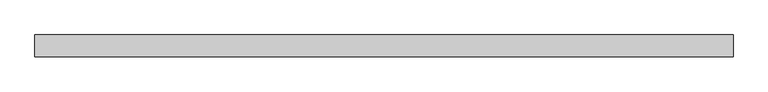
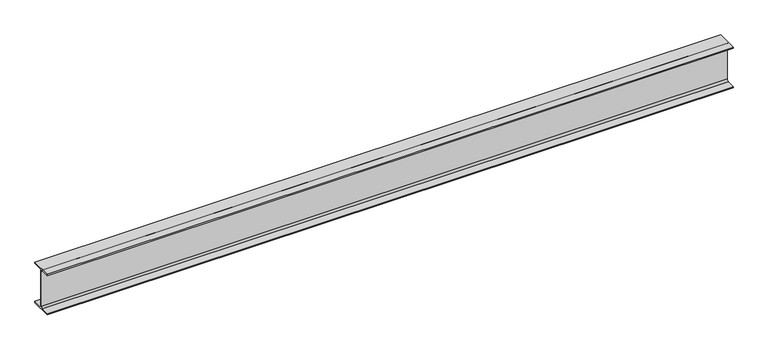
"""IFC4 building model written with IfcOpenShell, lengths in millimetres: beam geometry, 0912_Steel Framing_H-KSD3502 : H_SB_AR_S02_H-300x150x6.5x9_Stair."""

import ifcopenshell
import ifcopenshell.guid

model = None  # the IFC model being written
_history = None  # IfcOwnerHistory: only IFC2X3 demands one
_inside = {}  # id of a spatial element -> (the spatial element, [elements in it])
_under = {}  # id of a project, library or spatial element -> (it, [spatial elements below it])
_declared = {}  # id of a project -> (the project, [libraries it declares])
_typed = {}  # id of a type object -> (the type object, [elements of that type])
_made_of = {}  # id of a material, layer set ... -> (it, [elements and type objects made of it])


def new_model(schema):
    """Start an empty IFC model of exactly this schema.

    Asked for "IFC4X3", IfcOpenShell would pick the latest addendum, in which some entities
    have other attributes; the version numbers below select the first issue.
    IFC2X3 requires an IfcOwnerHistory on every rooted entity: one is made here for all.
    """
    global model, _history
    if schema == "IFC4X3":
        model = ifcopenshell.file(schema_version=(4, 3, 0, 0))
    else:
        model = ifcopenshell.file(schema=schema)
    _inside.clear()
    _under.clear()
    _declared.clear()
    _typed.clear()
    _made_of.clear()
    _history = None
    if model.schema == "IFC2X3":
        org = make("IfcOrganization", Name="unknown")
        user = make(
            "IfcPersonAndOrganization",
            ThePerson=make("IfcPerson", FamilyName="unknown"),
            TheOrganization=org,
        )
        app = make(
            "IfcApplication",
            ApplicationDeveloper=org,
            Version="unknown",
            ApplicationFullName="unknown",
            ApplicationIdentifier="unknown",
        )
        _history = make(
            "IfcOwnerHistory",
            OwningUser=user,
            OwningApplication=app,
            ChangeAction="ADDED",
            CreationDate=0,
        )
    return model


def make(cls, **values):
    """One entity of the class cls with the attributes given. An attribute that is None is left unset."""
    return model.create_entity(
        cls, **{name: value for name, value in values.items() if value is not None}
    )


def rooted(cls, **values):
    """An entity with a GlobalId (a new one), such as an element, a storey or a relation."""
    return make(cls, GlobalId=ifcopenshell.guid.new(), OwnerHistory=_history, **values)


def si_unit(unit_type, name, prefix=None):
    """IfcSIUnit, for example si_unit("LENGTHUNIT", "METRE", prefix="MILLI")."""
    return make("IfcSIUnit", UnitType=unit_type, Prefix=prefix, Name=name)


def assignment(units):
    """IfcUnitAssignment: the units of a project."""
    return None if units is None else make("IfcUnitAssignment", Units=units)


def point(xyz):
    """IfcCartesianPoint."""
    return None if xyz is None else make("IfcCartesianPoint", Coordinates=xyz)


def direction(xyz):
    """IfcDirection."""
    return None if xyz is None else make("IfcDirection", DirectionRatios=xyz)


def frame(location, z_axis=None, x_axis=None):
    """IfcAxis2Placement3D, a coordinate frame: its origin and axes. An axis left out is left unset."""
    return make(
        "IfcAxis2Placement3D",
        Location=point(location),
        Axis=direction(z_axis),
        RefDirection=direction(x_axis),
    )


def frame_2d(location, x_axis=None):
    """IfcAxis2Placement2D, a coordinate frame in the plane: its origin and x axis."""
    return make(
        "IfcAxis2Placement2D", Location=point(location), RefDirection=direction(x_axis)
    )


def origin():
    """The frame at (0, 0, 0) with its axes left unset."""
    return frame((0.0, 0.0, 0.0))


def place(relative_to, where):
    """IfcLocalPlacement: puts the frame where relative to a parent placement (None: the world)."""
    return make(
        "IfcLocalPlacement", PlacementRelTo=relative_to, RelativePlacement=where
    )


def context(
    kind, dimensions, precision=None, world=None, true_north=None, identifier=None
):
    """IfcGeometricRepresentationContext, for example the 3D "Model" context."""
    return make(
        "IfcGeometricRepresentationContext",
        ContextIdentifier=identifier,
        ContextType=kind,
        CoordinateSpaceDimension=dimensions,
        Precision=precision,
        WorldCoordinateSystem=world,
        TrueNorth=true_north,
    )


def project(units=None, contexts=None):
    """IfcProject with its units and contexts."""
    return rooted(
        "IfcProject",
        Name="project",
        RepresentationContexts=contexts,
        UnitsInContext=assignment(units),
    )


def spatial(cls, under=None, at=None, **own):
    """A site, building, storey or space (cls), placed at a placement, below another one or the project."""
    s = rooted(cls, ObjectPlacement=at, **own)
    if under is not None:
        _under.setdefault(under.id(), (under, []))[1].append(s)
    return s


def polyline(points):
    """IfcPolyline through the points."""
    return make("IfcPolyline", Points=[point(p) for p in points])


def circle_curve(where, radius):
    """IfcCircle in the frame where."""
    return make("IfcCircle", Position=where, Radius=radius)


def trimmed(basis, trim1, trim2, sense, master):
    """IfcTrimmedCurve: the piece of a basis curve between two trims."""
    return make(
        "IfcTrimmedCurve",
        BasisCurve=basis,
        Trim1=trim1,
        Trim2=trim2,
        SenseAgreement=sense,
        MasterRepresentation=master,
    )


def segment(curve, same_sense, transition):
    """IfcCompositeCurveSegment."""
    return make(
        "IfcCompositeCurveSegment",
        Transition=transition,
        SameSense=same_sense,
        ParentCurve=curve,
    )


def composite_curve(segments, self_intersect=None):
    """IfcCompositeCurve: segments joined end to end."""
    return make("IfcCompositeCurve", Segments=segments, SelfIntersect=self_intersect)


def outline(outer, holes=None, kind="AREA"):
    """IfcArbitraryClosedProfileDef: a profile drawn as a closed curve; with holes, ...WithVoids."""
    if holes is None:
        return make("IfcArbitraryClosedProfileDef", ProfileType=kind, OuterCurve=outer)
    return make(
        "IfcArbitraryProfileDefWithVoids",
        ProfileType=kind,
        OuterCurve=outer,
        InnerCurves=holes,
    )


def extrude(swept, where, along, depth):
    """IfcExtrudedAreaSolid: the profile swept, set in the frame where, extruded along a direction by depth."""
    return make(
        "IfcExtrudedAreaSolid",
        SweptArea=swept,
        Position=where,
        ExtrudedDirection=direction(along),
        Depth=depth,
    )


def shape(context_of_items, identifier, shape_type, items):
    """IfcShapeRepresentation: the items that make up one representation, for example the "Body"."""
    return make(
        "IfcShapeRepresentation",
        ContextOfItems=context_of_items,
        RepresentationIdentifier=identifier,
        RepresentationType=shape_type,
        Items=items,
    )


def source(mapping_origin, context_of_items, identifier, shape_type, items):
    """IfcRepresentationMap: a shape defined once, which mapped items show again and again."""
    return make(
        "IfcRepresentationMap",
        MappingOrigin=mapping_origin,
        MappedRepresentation=shape(context_of_items, identifier, shape_type, items),
    )


def transform(
    local_origin,
    x_axis=None,
    y_axis=None,
    z_axis=None,
    scale=None,
    scale2=None,
    scale3=None,
    uniform=True,
):
    """IfcCartesianTransformationOperator3D, or its non-uniform kind. x_axis, y_axis, z_axis: its Axis1, 2, 3."""
    if uniform:
        return make(
            "IfcCartesianTransformationOperator3D",
            Axis1=direction(x_axis),
            Axis2=direction(y_axis),
            LocalOrigin=point(local_origin),
            Scale=scale,
            Axis3=direction(z_axis),
        )
    return make(
        "IfcCartesianTransformationOperator3DnonUniform",
        Axis1=direction(x_axis),
        Axis2=direction(y_axis),
        LocalOrigin=point(local_origin),
        Scale=scale,
        Axis3=direction(z_axis),
        Scale2=scale2,
        Scale3=scale3,
    )


def mapped(mapping_source, mapping_target):
    """IfcMappedItem: shows the shape of a source again, moved by a transform."""
    return make(
        "IfcMappedItem", MappingSource=mapping_source, MappingTarget=mapping_target
    )


def made_of(thing, what):
    """Note that an element or type object is made of a material, layer set ...; save() writes the relation."""
    if what is not None:
        _made_of.setdefault(what.id(), (what, []))[1].append(thing)
    return thing


def element(
    cls,
    number,
    at=None,
    inside=None,
    cuts=None,
    type_object=None,
    material=None,
    context=None,
    identifier="Body",
    shape_type=None,
    held_by="IfcProductDefinitionShape",
    body=None,
    shapes=None,
    **own,
):
    """One element of the class cls, such as IfcWall. Its Tag is "e" and its number.

    at: its placement. inside: the storey or other place that contains it. cuts: it is an
    opening in that element (IfcRelVoidsElement). A single representation is given by context,
    identifier, shape_type and body (its items); several are given by shapes. held_by: the class
    of the entity that holds the representations. save() writes the other relations.
    """
    e = rooted(cls, Tag="e%d" % number, ObjectPlacement=at, **own)
    if body is not None:
        shapes = [shape(context, identifier, shape_type, body)]
    if shapes is not None:
        e.Representation = make(held_by, Representations=shapes)
    if inside is not None:
        _inside.setdefault(inside.id(), (inside, []))[1].append(e)
    if cuts is not None:
        rooted(
            "IfcRelVoidsElement", RelatingBuildingElement=cuts, RelatedOpeningElement=e
        )
    if type_object is not None:
        _typed.setdefault(type_object.id(), (type_object, []))[1].append(e)
    return made_of(e, material)


def aggregate(whole, parts):
    """IfcRelAggregates: a whole, such as a stair, and the parts it consists of."""
    return rooted("IfcRelAggregates", RelatingObject=whole, RelatedObjects=parts)


def save(model, path):
    """Write the relations noted so far, then the file.

    IfcRelAggregates (storeys below a building ...), IfcRelContainedInSpatialStructure (elements
    in a storey), IfcRelDefinesByType, IfcRelAssociatesMaterial and IfcRelDeclares: one each for
    every whole, place, type object, material and project.
    """
    for whole, parts in _under.values():
        aggregate(whole, parts)
    for where, things in _inside.values():
        rooted(
            "IfcRelContainedInSpatialStructure",
            RelatedElements=things,
            RelatingStructure=where,
        )
    for kind, things in _typed.values():
        rooted("IfcRelDefinesByType", RelatedObjects=things, RelatingType=kind)
    for what, things in _made_of.values():
        rooted("IfcRelAssociatesMaterial", RelatedObjects=things, RelatingMaterial=what)
    for by, libraries in _declared.values():
        rooted("IfcRelDeclares", RelatingContext=by, RelatedDefinitions=libraries)
    model.write(path)


def beam_fed367b4(model_context):
    return source(origin(), model_context, "Body", "SweptSolid", [
        extrude(outline(composite_curve([segment(polyline([(75.0, -141.0), (75.0, -150.0), (-75.0, -150.0), (-75.0, -141.0), (-16.25, -141.0)]), True, "CONTINUOUS"), segment(trimmed(circle_curve(frame_2d((-16.25, -128.0)), 13.0), [point((-16.25, -141.0))], [point((-3.25, -128.0))], True, "CARTESIAN"), True, "CONTINUOUS"), segment(polyline([(-3.25, -128.0), (-3.25, 128.0)]), True, "CONTINUOUS"), segment(trimmed(circle_curve(frame_2d((-16.25, 128.0)), 13.0), [point((-3.25, 128.0))], [point((-16.25, 141.0))], True, "CARTESIAN"), True, "CONTINUOUS"), segment(polyline([(-16.25, 141.0), (-75.0, 141.0), (-75.0, 150.0), (75.0, 150.0), (75.0, 141.0), (16.25, 141.0)]), True, "CONTINUOUS"), segment(trimmed(circle_curve(frame_2d((16.25, 128.0)), 13.0), [point((16.25, 141.0))], [point((3.25, 128.0))], True, "CARTESIAN"), True, "CONTINUOUS"), segment(polyline([(3.25, 128.0), (3.25, -128.0)]), True, "CONTINUOUS"), segment(trimmed(circle_curve(frame_2d((16.25, -128.0)), 13.0), [point((3.25, -128.0))], [point((16.25, -141.0))], True, "CARTESIAN"), True, "CONTINUOUS"), segment(polyline([(16.25, -141.0), (75.0, -141.0)]), True, "CONTINUOUS")], self_intersect=False)), frame((-2381.1079142, 0.0, 0.0), z_axis=(1.0, 0.0, 0.0), x_axis=(0.0, 1.0, 0.0)), (0.0, 0.0, 1.0), 4799.4668533),
    ])


if __name__ == "__main__":
    model = new_model("IFC4")
    model_context = context("Model", 3, world=origin())
    ifc_project = project(units=[si_unit("LENGTHUNIT", "METRE", prefix="MILLI")], contexts=[model_context])
    site = spatial("IfcSite", under=ifc_project)
    building = spatial("IfcBuilding", under=site)
    placement = place(None, origin())
    beam_shape = beam_fed367b4(model_context)
    element("IfcBeam", 1, ObjectType="0912_Steel Framing_H-KSD3502 : H_SB_AR_S02_H-300x150x6.5x9_Stair", at=placement, inside=building, context=model_context, shape_type="MappedRepresentation", body=[
        mapped(beam_shape, transform((0.0, 0.0, 0.0), x_axis=(1.0, 0.0, 0.0), y_axis=(0.0, 1.0, 0.0), z_axis=(0.0, 0.0, 1.0))),
    ])
    save(model, "model.ifc")

# Revit data of these elements
# Type "0912_Steel Framing_H-KSD3502 : H_SB_AR_S02_H-300x150x6.5x9_Stair"
#   H_Q'ty Cal Type Tag = "SB-Q2"
#   H_WM Code_1 = "S01AA073-00001 |  | TON | Main Steel Structure Fabrication Work | Shelter/Building | Medium Steel - Standard |  |  |  |  |  |  | Material: (   ) | (90)KG/M>Weight≥(30)KG/M | S01AA073-00001 Main Steel Structure Fabrication Work Shelter/Building Medium Steel - Standard         | - Material: ( ASTM A36 )\n- (90)KG/M>Weight≥(30)KG/M"
#   H_WM Code_2 = "S03AA083-00001 |  | TON | Main Steel Structure Erection Work | Shelter/Building | Medium Steel |  |  |  |  |  |  | Material: (   ) | S03AA083-00001 Main Steel Structure Erection Work Shelter/Building Medium Steel         | - Material: ( ASTM A36 )"
#   H_WM Code_3 = "S01AA009-00001 |  | TON | Main Steel Structure Fabrication Work | Shelter/Building | Plates - Gusset, Stiffener, ETC | Material: (   ) | S01AA009-00001 Main Steel Structure Fabrication Work Shelter/Building Plates - Gusset, Stiffener, ETC         |"
#   H_WM Code_4 = "S41AA051-00001 |  | M2 | Steel Structure Paint Work | Shelter/Building | for Non-Fireproofed Steel Surface |  |  |  |  |  |  | Material: (   ) | S41AA051-00001 Steel Structure Paint Work Shelter/Building for Non-Fireproofed Steel Surface         |"
#   Width = 15.0 cm
#   Web Thickness = 0.65 cm
#   Web Fillet = 1.3 cm
#   Warping Constant = 107000.0 cm⁶
#   W = 0
#   Torsional Moment of Inertia = 9.9539 cm⁴
#   Section Area = 46.78 cm²
#   Plastic Modulus weak axis = 105.0 cm³
#   Plastic Modulus strong axis = 542.0 cm³
#   Perimeter = 1.17 m²/m
#   Nominal Weight = 36.70 kgf/m
#   Moment of Inertia weak axis = 508.00 cm⁴
#   Moment of Inertia strong axis = 7210.00 cm⁴
#   Height = 30.0 cm
#   Flange Thickness = 0.9 cm
#   Elastic Modulus weak axis = 67.7 cm³
#   Elastic Modulus strong axis = 481.0 cm³
#   Centroid Vertical = 15.0 cm
#   Centroid Horizontal = 7.5 cm
#   Ix = 72100000
#   Length [instance default] = 1524 mm
#   Zx = 542000
#   b = 150 mm
#   h = 300 mm
#   r = 13 mm
#   s = 6.5 mm
#   t = 9 mm
#   A = 0.004678 m²
#   Structural Material [instance default] = Steel, 45-345
#   Assembly Code = ""
# Element 1 (IfcBeam, "0912_Steel Framing_H-KSD3502 : H_SB_AR_S02_H-300x150x6.5x9_Stair")
#   Materials on its faces: "Steel, 45-345"
# Materials
#   "Steel, 45-345": class "Metal", colour RGB 189 187 185, transparency 0, Description = "Steel 345 MPa", Cost = 0
